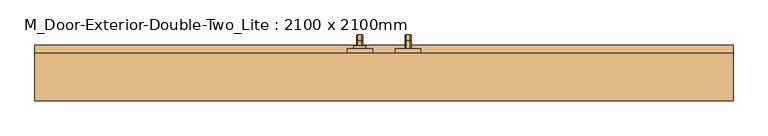
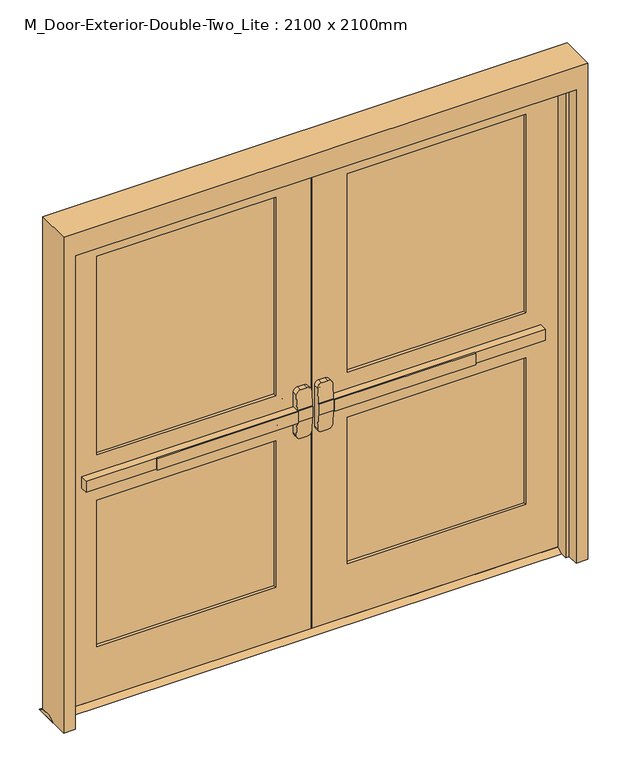
"""IFC4 building model written with IfcOpenShell, lengths in millimetres: door geometry, M_Door-Exterior-Double-Two_Lite : 2100 x 2100mm."""

from ifc_helpers import new_model, si_unit, point, frame, frame_2d, origin, place, context, project, spatial, polyline, circle_curve, ellipse_curve, trimmed, segment, composite_curve, outline, extrude, faceted_brep, source, transform, mapped, element, save
from ifc_brep_helpers import plane_surface, cylinder_surface, revolved_surface, advanced_brep


def m_door_exterior_double_two_lite_2100_x_2100mm_462d4e28(model_context):
    return source(origin(), model_context, "Body", "SolidModel", [
        extrude(outline(polyline([(-667.2, -39.25), (-667.2, -32.9), (-76.2, -32.9), (-76.2, -39.25), (-667.2, -39.25)])), frame((0.0, 0.0, 974.6), z_axis=(0.0, 0.0, 1.0), x_axis=(1.0, 0.0, 0.0)), (0.0, 0.0, 1.0), 50.8),
        advanced_brep(
        [(-12.7, -32.9, 1025.4), (-76.2, -32.9, 1025.4), (-962.7, -32.9, 1025.4), (-962.7, -32.9, 974.6), (-76.2, -32.9, 974.6), (-12.7, -32.9, 974.6), (-962.7, -1.15, 1025.4), (-76.2, -1.15, 1025.4), (-76.2, -1.15, 1088.9), (-57.15, -1.15, 1107.95), (-31.75, -1.15, 1107.95), (-12.7, -1.15, 1088.9), (-12.7, -1.15, 911.1), (-31.75, -1.15, 892.05), (-57.15, -1.15, 892.05), (-76.2, -1.15, 911.1), (-76.2, -1.15, 974.6), (-962.7, -1.15, 974.6), (-12.7, -29.7247533, 1025.4), (-76.2, -29.7247533, 1025.4), (-12.7, -29.7247533, 974.6), (-12.7, -24.7145731, 911.1), (-12.7, -24.7145731, 1088.9), (-76.2, -29.7247533, 974.6), (-76.2, -24.7145731, 1088.9), (-76.2, -24.7145731, 911.1), (-57.15, -23.211519, 1107.95), (-31.75, -23.211519, 1107.95), (-31.75, -23.211519, 892.05), (-57.15, -23.211519, 892.05)],
        [
            (0, 1),
            (1, 2),
            (2, 3),
            (3, 4),
            (4, 5),
            (5, 0),
            (6, 7),
            (7, 8),
            (8, 9, circle_curve(frame((-57.15, -1.15, 1088.9), z_axis=(0.0, 1.0, 0.0), x_axis=(-1.0, 0.0, 0.0)), 19.05)),
            (9, 10),
            (10, 11, circle_curve(frame((-31.75, -1.15, 1088.9), z_axis=(0.0, 1.0, 0.0), x_axis=(-1.0, 0.0, 0.0)), 19.05)),
            (11, 12),
            (12, 13, circle_curve(frame((-31.75, -1.15, 911.1), z_axis=(0.0, 1.0, 0.0), x_axis=(-1.0, 0.0, 0.0)), 19.05)),
            (13, 14),
            (14, 15, circle_curve(frame((-57.15, -1.15, 911.1), z_axis=(0.0, 1.0, 0.0), x_axis=(-1.0, 0.0, 0.0)), 19.05)),
            (15, 16),
            (16, 17),
            (17, 6),
            (0, 18),
            (18, 19),
            (19, 7),
            (6, 2),
            (5, 20),
            (20, 21),
            (21, 12),
            (11, 22),
            (22, 18),
            (16, 23),
            (23, 20),
            (3, 17),
            (19, 24),
            (24, 8),
            (15, 25),
            (25, 23),
            (9, 26),
            (26, 27),
            (27, 10),
            (13, 28),
            (28, 29),
            (29, 14),
            (29, 25, ellipse_curve(frame((-57.15, -24.7145731, 911.1), z_axis=(0.0, 0.9969018152893365, 0.07865602756830282), x_axis=(0.0, -0.07865602756830208, 0.9969018152893365)), 19.1092038, 19.05)),
            (24, 26, ellipse_curve(frame((-57.15, -24.7145731, 1088.9), z_axis=(0.0, 0.9969018152893376, -0.07865602756828934), x_axis=(0.0, -0.078656027568288, -0.9969018152893377)), 19.1092038, 19.05)),
            (27, 22, ellipse_curve(frame((-31.75, -24.7145731, 1088.9), z_axis=(0.0, 0.9969018152893376, -0.07865602756828934), x_axis=(0.0, -0.078656027568288, -0.9969018152893377)), 19.1092038, 19.05)),
            (21, 28, ellipse_curve(frame((-31.75, -24.7145731, 911.1), z_axis=(0.0, 0.9969018152893365, 0.07865602756830282), x_axis=(0.0, -0.07865602756830208, 0.9969018152893365)), 19.1092038, 19.05)),
        ],
        [
            plane_surface(frame((-12.7, -32.9, 1025.4), z_axis=(0.0, -1.0, 0.0), x_axis=(1.0, 0.0, 0.0))),
            plane_surface(frame((-12.7, -1.15, 1025.4), z_axis=(0.0, 1.0, 0.0), x_axis=(-1.0, 0.0, 0.0))),
            plane_surface(frame((-962.7, -32.9, 1025.4), z_axis=(0.0, 0.0, 1.0), x_axis=(0.0, 1.0, 0.0))),
            plane_surface(frame((-12.7, -32.9, 1025.4), z_axis=(1.0, 0.0, 0.0), x_axis=(0.0, 1.0, 0.0))),
            plane_surface(frame((-12.7, -32.9, 974.6), z_axis=(0.0, 0.0, -1.0), x_axis=(0.0, 1.0, 0.0))),
            plane_surface(frame((-962.7, -32.9, 974.6), z_axis=(-1.0, 0.0, 0.0), x_axis=(0.0, 1.0, 0.0))),
            plane_surface(frame((-76.2, -29.7247533, 911.1), z_axis=(-1.0, 0.0, 0.0), x_axis=(0.0, 1.0, 0.0))),
            plane_surface(frame((-57.15, -29.7247533, 1107.95), z_axis=(0.0, 0.0, 1.0), x_axis=(0.0, 1.0, 0.0))),
            plane_surface(frame((-31.75, -29.7247533, 892.05), z_axis=(0.0, 0.0, -1.0), x_axis=(0.0, 1.0, 0.0))),
            cylinder_surface(frame((-57.15, -1.15, 911.1), z_axis=(0.0, -1.0, 0.0), x_axis=(-1.0, 0.0, 0.0)), 19.05),
            cylinder_surface(frame((-57.15, -1.15, 1088.9), z_axis=(0.0, -1.0, 0.0), x_axis=(-1.0, 0.0, 0.0)), 19.05),
            cylinder_surface(frame((-31.75, -1.15, 1088.9), z_axis=(0.0, -1.0, 0.0), x_axis=(-1.0, 0.0, 0.0)), 19.05),
            cylinder_surface(frame((-31.75, -1.15, 911.1), z_axis=(0.0, -1.0, 0.0), x_axis=(-1.0, 0.0, 0.0)), 19.05),
            plane_surface(frame((-76.2, -29.7247533, 1025.4), z_axis=(0.0, -0.9969018152893376, 0.07865602756828934), x_axis=(1.0, 0.0, 0.0))),
            plane_surface(frame((-76.2, -23.211519, 892.05), z_axis=(0.0, -0.9969018152893365, -0.07865602756830282), x_axis=(1.0, 0.0, 0.0))),
        ],
        [
            (0, [[1, 2, 3, 4, 5, 6]]),
            (1, [[7, 8, 9, 10, 11, 12, 13, 14, 15, 16, 17, 18]]),
            (2, [[-2, -1, 19, 20, 21, -7, 22]]),
            (3, [[23, 24, 25, -12, 26, 27, -19, -6]]),
            (4, [[-17, 28, 29, -23, -5, -4, 30]]),
            (5, [[-22, -18, -30, -3]]),
            (6, [[-21, 31, 32, -8]]),
            (6, [[33, 34, -28, -16]]),
            (7, [[35, 36, 37, -10]]),
            (8, [[38, 39, 40, -14]]),
            (9, [[-40, 41, -33, -15]]),
            (10, [[-32, 42, -35, -9]]),
            (11, [[-37, 43, -26, -11]]),
            (12, [[-25, 44, -38, -13]]),
            (13, [[-27, -43, -36, -42, -31, -20]]),
            (14, [[-29, -34, -41, -39, -44, -24]]),
        ],
    ),
        extrude(outline(polyline([(43.85, 15.0), (69.25, 0.0), (-26.55, 0.0), (-1.15, 15.0), (43.85, 15.0)])), frame((-1100.0, 0.0, 0.0), z_axis=(1.0, 0.0, 0.0), x_axis=(0.0, 1.0, 0.0)), (0.0, 0.0, 1.0), 2200.0),
        extrude(outline(polyline([(667.2, -39.25), (76.2, -39.25), (76.2, -32.9), (667.2, -32.9), (667.2, -39.25)])), frame((0.0, 0.0, 974.6), z_axis=(0.0, 0.0, 1.0), x_axis=(1.0, 0.0, 0.0)), (0.0, 0.0, 1.0), 50.8),
        advanced_brep(
        [(12.7, -32.9, 1025.4), (12.7, -32.9, 974.6), (76.2, -32.9, 974.6), (962.7, -32.9, 974.6), (962.7, -32.9, 1025.4), (76.2, -32.9, 1025.4), (962.7, -1.15, 1025.4), (962.7, -1.15, 974.6), (76.2, -1.15, 974.6), (76.2, -1.15, 911.1), (57.15, -1.15, 892.05), (31.75, -1.15, 892.05), (12.7, -1.15, 911.1), (12.7, -1.15, 1088.9), (31.75, -1.15, 1107.95), (57.15, -1.15, 1107.95), (76.2, -1.15, 1088.9), (76.2, -1.15, 1025.4), (76.2, -29.7247533, 1025.4), (12.7, -29.7247533, 1025.4), (12.7, -24.7145731, 1088.9), (12.7, -24.7145731, 911.1), (12.7, -29.7247533, 974.6), (76.2, -29.7247533, 974.6), (76.2, -24.7145731, 911.1), (76.2, -24.7145731, 1088.9), (31.75, -23.211519, 1107.95), (57.15, -23.211519, 1107.95), (57.15, -23.211519, 892.05), (31.75, -23.211519, 892.05)],
        [
            (0, 1),
            (1, 2),
            (2, 3),
            (3, 4),
            (4, 5),
            (5, 0),
            (6, 7),
            (7, 8),
            (8, 9),
            (9, 10, circle_curve(frame((57.15, -1.15, 911.1), z_axis=(0.0, 1.0, 0.0), x_axis=(1.0, 0.0, 0.0)), 19.05)),
            (10, 11),
            (11, 12, circle_curve(frame((31.75, -1.15, 911.1), z_axis=(0.0, 1.0, 0.0), x_axis=(1.0, 0.0, 0.0)), 19.05)),
            (12, 13),
            (13, 14, circle_curve(frame((31.75, -1.15, 1088.9), z_axis=(0.0, 1.0, 0.0), x_axis=(1.0, 0.0, 0.0)), 19.05)),
            (14, 15),
            (15, 16, circle_curve(frame((57.15, -1.15, 1088.9), z_axis=(0.0, 1.0, 0.0), x_axis=(1.0, 0.0, 0.0)), 19.05)),
            (16, 17),
            (17, 6),
            (4, 6),
            (17, 18),
            (18, 19),
            (19, 0),
            (19, 20),
            (20, 13),
            (12, 21),
            (21, 22),
            (22, 1),
            (7, 3),
            (22, 23),
            (23, 8),
            (23, 24),
            (24, 9),
            (16, 25),
            (25, 18),
            (14, 26),
            (26, 27),
            (27, 15),
            (10, 28),
            (28, 29),
            (29, 11),
            (24, 28, ellipse_curve(frame((57.15, -24.7145731, 911.1), z_axis=(0.0, 0.9969018152893365, 0.07865602756830282), x_axis=(0.0, -0.07865602756830208, 0.9969018152893365)), 19.1092038, 19.05)),
            (27, 25, ellipse_curve(frame((57.15, -24.7145731, 1088.9), z_axis=(0.0, 0.9969018152893376, -0.07865602756828934), x_axis=(0.0, -0.078656027568288, -0.9969018152893377)), 19.1092038, 19.05)),
            (20, 26, ellipse_curve(frame((31.75, -24.7145731, 1088.9), z_axis=(0.0, 0.9969018152893376, -0.07865602756828934), x_axis=(0.0, -0.078656027568288, -0.9969018152893377)), 19.1092038, 19.05)),
            (29, 21, ellipse_curve(frame((31.75, -24.7145731, 911.1), z_axis=(0.0, 0.9969018152893365, 0.07865602756830282), x_axis=(0.0, -0.07865602756830208, 0.9969018152893365)), 19.1092038, 19.05)),
        ],
        [
            plane_surface(frame((12.7, -32.9, 1025.4), z_axis=(0.0, -1.0, 0.0), x_axis=(-1.0, 0.0, 0.0))),
            plane_surface(frame((12.7, -1.15, 1025.4), z_axis=(0.0, 1.0, 0.0), x_axis=(1.0, 0.0, 0.0))),
            plane_surface(frame((962.7, -32.9, 1025.4), z_axis=(0.0, 0.0, 1.0), x_axis=(0.0, 1.0, 0.0))),
            plane_surface(frame((12.7, -32.9, 1025.4), z_axis=(-1.0, 0.0, 0.0), x_axis=(0.0, 1.0, 0.0))),
            plane_surface(frame((12.7, -32.9, 974.6), z_axis=(0.0, 0.0, -1.0), x_axis=(0.0, 1.0, 0.0))),
            plane_surface(frame((962.7, -32.9, 974.6), z_axis=(1.0, 0.0, 0.0), x_axis=(0.0, 1.0, 0.0))),
            plane_surface(frame((76.2, -29.7247533, 911.1), z_axis=(1.0, 0.0, 0.0), x_axis=(0.0, 1.0, 0.0))),
            plane_surface(frame((57.15, -29.7247533, 1107.95), z_axis=(0.0, 0.0, 1.0), x_axis=(0.0, 1.0, 0.0))),
            plane_surface(frame((31.75, -29.7247533, 892.05), z_axis=(0.0, 0.0, -1.0), x_axis=(0.0, 1.0, 0.0))),
            cylinder_surface(frame((57.15, -1.15, 911.1), z_axis=(0.0, -1.0, 0.0), x_axis=(1.0, 0.0, 0.0)), 19.05),
            cylinder_surface(frame((57.15, -1.15, 1088.9), z_axis=(0.0, -1.0, 0.0), x_axis=(1.0, 0.0, 0.0)), 19.05),
            cylinder_surface(frame((31.75, -1.15, 1088.9), z_axis=(0.0, -1.0, 0.0), x_axis=(1.0, 0.0, 0.0)), 19.05),
            cylinder_surface(frame((31.75, -1.15, 911.1), z_axis=(0.0, -1.0, 0.0), x_axis=(1.0, 0.0, 0.0)), 19.05),
            plane_surface(frame((76.2, -29.7247533, 1025.4), z_axis=(0.0, -0.9969018152893376, 0.07865602756828934), x_axis=(-1.0, 0.0, 0.0))),
            plane_surface(frame((76.2, -23.211519, 892.05), z_axis=(0.0, -0.9969018152893365, -0.07865602756830282), x_axis=(-1.0, 0.0, 0.0))),
        ],
        [
            (0, [[1, 2, 3, 4, 5, 6]]),
            (1, [[7, 8, 9, 10, 11, 12, 13, 14, 15, 16, 17, 18]]),
            (2, [[19, -18, 20, 21, 22, -6, -5]]),
            (3, [[-1, -22, 23, 24, -13, 25, 26, 27]]),
            (4, [[28, -3, -2, -27, 29, 30, -8]]),
            (5, [[-4, -28, -7, -19]]),
            (6, [[-9, -30, 31, 32]]),
            (6, [[-17, 33, 34, -20]]),
            (7, [[-15, 35, 36, 37]]),
            (8, [[-11, 38, 39, 40]]),
            (9, [[-10, -32, 41, -38]]),
            (10, [[-16, -37, 42, -33]]),
            (11, [[-14, -24, 43, -35]]),
            (12, [[-12, -40, 44, -25]]),
            (13, [[-21, -34, -42, -36, -43, -23]]),
            (14, [[-26, -44, -39, -41, -31, -29]]),
        ],
    ),
        advanced_brep(
        [(66.2, 58.85, 1001.190625), (66.2, 58.85, 998.809375), (69.771875, 58.85, 995.2375), (82.6284594, 58.85, 995.2375), (86.2, 58.85, 998.8090406), (86.2, 58.85, 1001.190625), (82.628125, 58.85, 1004.7625), (69.771875, 58.85, 1004.7625), (66.2, 58.85, 874.609375), (69.771875, 58.85, 871.0375), (82.628125, 58.85, 871.0375), (86.2, 58.85, 874.609375), (86.2, 58.85, 876.9909594), (82.6284594, 58.85, 880.5625), (69.771875, 58.85, 880.5625), (66.2, 58.85, 876.990625), (66.2, 84.25, 1001.190625), (66.2, 98.140625, 987.3), (66.2, 98.140625, 888.5), (66.2, 84.25, 874.609375), (66.2, 84.25, 876.990625), (66.2, 95.759375, 888.5), (66.2, 95.759375, 987.3), (66.2, 84.25, 998.809375), (69.771875, 84.25, 995.2375), (82.6284594, 84.25, 995.2375), (86.2, 84.25, 998.8090406), (86.2, 95.7590406, 987.3), (86.2, 95.7590406, 888.5), (86.2, 84.25, 876.9909594), (86.2, 84.25, 874.609375), (86.2, 98.140625, 888.5), (86.2, 98.140625, 987.3), (86.2, 84.25, 1001.190625), (82.628125, 84.25, 1004.7625), (69.771875, 84.25, 1004.7625), (69.771875, 92.1875, 987.3), (82.6284594, 92.1875, 987.3), (82.628125, 101.7125, 987.3), (69.771875, 101.7125, 987.3), (69.771875, 92.1875, 888.5), (82.6284594, 92.1875, 888.5), (82.628125, 101.7125, 888.5), (69.771875, 101.7125, 888.5), (69.771875, 84.25, 880.5625), (82.6284594, 84.25, 880.5625), (82.628125, 84.25, 871.0375), (69.771875, 84.25, 871.0375)],
        [
            (0, 1),
            (1, 2, circle_curve(frame((69.771875, 58.85, 998.809375), z_axis=(0.0, -1.0, 0.0), x_axis=(0.0, 0.0, 1.0)), 3.571875)),
            (2, 3),
            (3, 4, circle_curve(frame((82.6284594, 58.85, 998.8090406), z_axis=(0.0, -1.0, 0.0), x_axis=(0.0, 0.0, 1.0)), 3.5715406)),
            (4, 5),
            (5, 6, circle_curve(frame((82.628125, 58.85, 1001.190625), z_axis=(0.0, -1.0, 0.0), x_axis=(0.0, 0.0, 1.0)), 3.571875)),
            (6, 7),
            (7, 0, circle_curve(frame((69.771875, 58.85, 1001.190625), z_axis=(0.0, -1.0, 0.0), x_axis=(0.0, 0.0, 1.0)), 3.571875)),
            (8, 9, circle_curve(frame((69.771875, 58.85, 874.609375), z_axis=(0.0, -1.0, 0.0), x_axis=(0.0, 0.0, -1.0)), 3.571875)),
            (9, 10),
            (10, 11, circle_curve(frame((82.628125, 58.85, 874.609375), z_axis=(0.0, -1.0, 0.0), x_axis=(0.0, 0.0, -1.0)), 3.571875)),
            (11, 12),
            (12, 13, circle_curve(frame((82.6284594, 58.85, 876.9909594), z_axis=(0.0, -1.0, 0.0), x_axis=(0.0, 0.0, -1.0)), 3.5715406)),
            (13, 14),
            (14, 15, circle_curve(frame((69.771875, 58.85, 876.990625), z_axis=(0.0, -1.0, 0.0), x_axis=(0.0, 0.0, -1.0)), 3.571875)),
            (15, 8),
            (0, 16),
            (16, 17, circle_curve(frame((66.2, 84.25, 987.3), z_axis=(-1.0, 0.0, 0.0), x_axis=(0.0, 0.0, 1.0)), 13.890625)),
            (17, 18),
            (18, 19, circle_curve(frame((66.2, 84.25, 888.5), z_axis=(-1.0, 0.0, 0.0), x_axis=(0.0, 1.0, 0.0)), 13.890625)),
            (19, 8),
            (15, 20),
            (20, 21, circle_curve(frame((66.2, 84.25, 888.5), z_axis=(1.0, 0.0, 0.0), x_axis=(0.0, 1.0, 0.0)), 11.509375)),
            (21, 22),
            (22, 23, circle_curve(frame((66.2, 84.25, 987.3), z_axis=(1.0, 0.0, 0.0), x_axis=(0.0, 0.0, 1.0)), 11.509375)),
            (23, 1),
            (23, 24, circle_curve(frame((69.771875, 84.25, 998.809375), z_axis=(0.0, -1.0, 0.0), x_axis=(0.0, 0.0, 1.0)), 3.571875)),
            (24, 2),
            (24, 25),
            (25, 3),
            (25, 26, circle_curve(frame((82.6284594, 84.25, 998.8090406), z_axis=(0.0, -1.0, 0.0), x_axis=(0.0, 0.0, 1.0)), 3.5715406)),
            (26, 4),
            (26, 27, circle_curve(frame((86.2, 84.25, 987.3), z_axis=(-1.0, 0.0, 0.0), x_axis=(0.0, 0.0, 1.0)), 11.5090406)),
            (27, 28),
            (28, 29, circle_curve(frame((86.2, 84.25, 888.5), z_axis=(-1.0, 0.0, 0.0), x_axis=(0.0, 1.0, 0.0)), 11.5090406)),
            (29, 12),
            (11, 30),
            (30, 31, circle_curve(frame((86.2, 84.25, 888.5), z_axis=(1.0, 0.0, 0.0), x_axis=(0.0, 1.0, 0.0)), 13.890625)),
            (31, 32),
            (32, 33, circle_curve(frame((86.2, 84.25, 987.3), z_axis=(1.0, 0.0, 0.0), x_axis=(0.0, 0.0, 1.0)), 13.890625)),
            (33, 5),
            (33, 34, circle_curve(frame((82.628125, 84.25, 1001.190625), z_axis=(0.0, -1.0, 0.0), x_axis=(0.0, 0.0, 1.0)), 3.571875)),
            (34, 6),
            (34, 35),
            (35, 7),
            (35, 16, circle_curve(frame((69.771875, 84.25, 1001.190625), z_axis=(0.0, -1.0, 0.0), x_axis=(0.0, 0.0, 1.0)), 3.571875)),
            (36, 24, circle_curve(frame((69.771875, 84.25, 987.3), z_axis=(1.0, 0.0, 0.0), x_axis=(0.0, 0.0, 1.0)), 7.9375)),
            (22, 36, circle_curve(frame((69.771875, 95.759375, 987.3), z_axis=(0.0, 0.0, 1.0), x_axis=(0.0, 1.0, 0.0)), 3.571875)),
            (37, 25, circle_curve(frame((82.6284594, 84.25, 987.3), z_axis=(1.0, 0.0, 0.0), x_axis=(0.0, 0.0, 1.0)), 7.9375)),
            (36, 37),
            (37, 27, circle_curve(frame((82.6284594, 95.7590406, 987.3), z_axis=(0.0, 0.0, 1.0), x_axis=(0.0, 1.0, 0.0)), 3.5715406)),
            (38, 34, circle_curve(frame((82.628125, 84.25, 987.3), z_axis=(1.0, 0.0, 0.0), x_axis=(0.0, 0.0, 1.0)), 17.4625)),
            (32, 38, circle_curve(frame((82.628125, 98.140625, 987.3), z_axis=(0.0, 0.0, 1.0), x_axis=(0.0, 1.0, 0.0)), 3.571875)),
            (39, 35, circle_curve(frame((69.771875, 84.25, 987.3), z_axis=(1.0, 0.0, 0.0), x_axis=(0.0, 0.0, 1.0)), 17.4625)),
            (38, 39),
            (39, 17, circle_curve(frame((69.771875, 98.140625, 987.3), z_axis=(0.0, 0.0, 1.0), x_axis=(0.0, 1.0, 0.0)), 3.571875)),
            (21, 40, circle_curve(frame((69.771875, 95.759375, 888.5), z_axis=(0.0, 0.0, 1.0), x_axis=(0.0, 1.0, 0.0)), 3.571875)),
            (40, 36),
            (40, 41),
            (41, 37),
            (41, 28, circle_curve(frame((82.6284594, 95.7590406, 888.5), z_axis=(0.0, 0.0, 1.0), x_axis=(0.0, 1.0, 0.0)), 3.5715406)),
            (31, 42, circle_curve(frame((82.628125, 98.140625, 888.5), z_axis=(0.0, 0.0, 1.0), x_axis=(0.0, 1.0, 0.0)), 3.571875)),
            (42, 38),
            (42, 43),
            (43, 39),
            (43, 18, circle_curve(frame((69.771875, 98.140625, 888.5), z_axis=(0.0, 0.0, 1.0), x_axis=(0.0, 1.0, 0.0)), 3.571875)),
            (44, 40, circle_curve(frame((69.771875, 84.25, 888.5), z_axis=(1.0, 0.0, 0.0), x_axis=(0.0, 1.0, 0.0)), 7.9375)),
            (20, 44, circle_curve(frame((69.771875, 84.25, 876.990625), z_axis=(0.0, 1.0, 0.0), x_axis=(0.0, 0.0, -1.0)), 3.571875)),
            (45, 41, circle_curve(frame((82.6284594, 84.25, 888.5), z_axis=(1.0, 0.0, 0.0), x_axis=(0.0, 1.0, 0.0)), 7.9375)),
            (44, 45),
            (45, 29, circle_curve(frame((82.6284594, 84.25, 876.9909594), z_axis=(0.0, 1.0, 0.0), x_axis=(0.0, 0.0, -1.0)), 3.5715406)),
            (46, 42, circle_curve(frame((82.628125, 84.25, 888.5), z_axis=(1.0, 0.0, 0.0), x_axis=(0.0, 1.0, 0.0)), 17.4625)),
            (30, 46, circle_curve(frame((82.628125, 84.25, 874.609375), z_axis=(0.0, 1.0, 0.0), x_axis=(0.0, 0.0, -1.0)), 3.571875)),
            (47, 43, circle_curve(frame((69.771875, 84.25, 888.5), z_axis=(1.0, 0.0, 0.0), x_axis=(0.0, 1.0, 0.0)), 17.4625)),
            (46, 47),
            (47, 19, circle_curve(frame((69.771875, 84.25, 874.609375), z_axis=(0.0, 1.0, 0.0), x_axis=(0.0, 0.0, -1.0)), 3.571875)),
            (14, 44),
            (13, 45),
            (10, 46),
            (9, 47),
        ],
        [
            plane_surface(frame((76.2, 58.85, 1000.0), z_axis=(0.0, -1.0, 0.0), x_axis=(1.0, 0.0, 0.0))),
            plane_surface(frame((76.2, 58.85, 875.8), z_axis=(0.0, -1.0, 0.0), x_axis=(1.0, 0.0, 0.0))),
            plane_surface(frame((66.2, 58.85, 1001.190625), z_axis=(-1.0, 0.0, 0.0), x_axis=(0.0, 1.0, 0.0))),
            cylinder_surface(frame((69.771875, 58.85, 998.809375), z_axis=(0.0, -1.0, 0.0), x_axis=(0.0, 0.0, 1.0)), 3.571875),
            plane_surface(frame((69.771875, 58.85, 995.2375), z_axis=(0.0, 0.0, -1.0), x_axis=(0.0, 1.0, 0.0))),
            cylinder_surface(frame((82.6284594, 58.85, 998.8090406), z_axis=(0.0, -1.0, 0.0), x_axis=(0.0, 0.0, 1.0)), 3.5715406),
            plane_surface(frame((86.2, 58.85, 998.8090406), z_axis=(1.0, 0.0, 0.0), x_axis=(0.0, 1.0, 0.0))),
            cylinder_surface(frame((82.628125, 58.85, 1001.190625), z_axis=(0.0, -1.0, 0.0), x_axis=(0.0, 0.0, 1.0)), 3.571875),
            plane_surface(frame((82.628125, 58.85, 1004.7625), z_axis=(0.0, 0.0, 1.0), x_axis=(0.0, 1.0, 0.0))),
            cylinder_surface(frame((69.771875, 58.85, 1001.190625), z_axis=(0.0, -1.0, 0.0), x_axis=(0.0, 0.0, 1.0)), 3.571875),
            revolved_surface(trimmed(ellipse_curve(frame((69.771875, 84.25, 998.809375), z_axis=(0.0, -1.0, 0.0), x_axis=(0.0, 0.0, 1.0)), 3.571875, 3.571875), [point((66.2, 84.25, 998.809375))], [point((69.771875, 84.25, 995.2375))], True, "CARTESIAN"), (76.2, 84.25, 987.3), (-1.0, 0.0, 0.0)),
            revolved_surface(polyline([(69.771875, 84.25, 995.2375), (82.6284594, 84.25, 995.2375)]), (76.2, 84.25, 987.3), (-1.0, 0.0, 0.0)),
            revolved_surface(trimmed(ellipse_curve(frame((82.6284594, 84.25, 998.8090406), z_axis=(0.0, -1.0, 0.0), x_axis=(0.0, 0.0, 1.0)), 3.5715406, 3.5715406), [point((82.6284594, 84.25, 995.2375))], [point((86.2, 84.25, 998.8090406))], True, "CARTESIAN"), (76.2, 84.25, 987.3), (-1.0, 0.0, 0.0)),
            revolved_surface(trimmed(ellipse_curve(frame((82.628125, 84.25, 1001.190625), z_axis=(0.0, -1.0, 0.0), x_axis=(0.0, 0.0, 1.0)), 3.571875, 3.571875), [point((86.2, 84.25, 1001.190625))], [point((82.628125, 84.25, 1004.7625))], True, "CARTESIAN"), (76.2, 84.25, 987.3), (-1.0, 0.0, 0.0)),
            cylinder_surface(frame((76.2, 84.25, 987.3), z_axis=(-1.0, 0.0, 0.0), x_axis=(0.0, 0.0, 1.0)), 17.4625),
            revolved_surface(trimmed(ellipse_curve(frame((69.771875, 84.25, 1001.190625), z_axis=(0.0, -1.0, 0.0), x_axis=(0.0, 0.0, 1.0)), 3.571875, 3.571875), [point((69.771875, 84.25, 1004.7625))], [point((66.2, 84.25, 1001.190625))], True, "CARTESIAN"), (76.2, 84.25, 987.3), (-1.0, 0.0, 0.0)),
            cylinder_surface(frame((69.771875, 95.759375, 987.3), z_axis=(0.0, 0.0, 1.0), x_axis=(0.0, 1.0, 0.0)), 3.571875),
            plane_surface(frame((69.771875, 92.1875, 987.3), z_axis=(0.0, -1.0, 0.0), x_axis=(0.0, 0.0, -1.0))),
            cylinder_surface(frame((82.6284594, 95.7590406, 987.3), z_axis=(0.0, 0.0, 1.0), x_axis=(0.0, 1.0, 0.0)), 3.5715406),
            cylinder_surface(frame((82.628125, 98.140625, 987.3), z_axis=(0.0, 0.0, 1.0), x_axis=(0.0, 1.0, 0.0)), 3.571875),
            plane_surface(frame((82.628125, 101.7125, 987.3), z_axis=(0.0, 1.0, 0.0), x_axis=(0.0, 0.0, -1.0))),
            cylinder_surface(frame((69.771875, 98.140625, 987.3), z_axis=(0.0, 0.0, 1.0), x_axis=(0.0, 1.0, 0.0)), 3.571875),
            revolved_surface(trimmed(ellipse_curve(frame((69.771875, 95.759375, 888.5), z_axis=(0.0, 0.0, 1.0), x_axis=(0.0, 1.0, 0.0)), 3.571875, 3.571875), [point((66.2, 95.759375, 888.5))], [point((69.771875, 92.1875, 888.5))], True, "CARTESIAN"), (76.2, 84.25, 888.5), (-1.0, 0.0, 0.0)),
            revolved_surface(polyline([(69.771875, 92.1875, 888.5), (82.6284594, 92.1875, 888.5)]), (76.2, 84.25, 888.5), (-1.0, 0.0, 0.0)),
            revolved_surface(trimmed(ellipse_curve(frame((82.6284594, 95.7590406, 888.5), z_axis=(0.0, 0.0, 1.0), x_axis=(0.0, 1.0, 0.0)), 3.5715406, 3.5715406), [point((82.6284594, 92.1875, 888.5))], [point((86.2, 95.7590406, 888.5))], True, "CARTESIAN"), (76.2, 84.25, 888.5), (-1.0, 0.0, 0.0)),
            revolved_surface(trimmed(ellipse_curve(frame((82.628125, 98.140625, 888.5), z_axis=(0.0, 0.0, 1.0), x_axis=(0.0, 1.0, 0.0)), 3.571875, 3.571875), [point((86.2, 98.140625, 888.5))], [point((82.628125, 101.7125, 888.5))], True, "CARTESIAN"), (76.2, 84.25, 888.5), (-1.0, 0.0, 0.0)),
            cylinder_surface(frame((76.2, 84.25, 888.5), z_axis=(-1.0, 0.0, 0.0), x_axis=(0.0, 1.0, 0.0)), 17.4625),
            revolved_surface(trimmed(ellipse_curve(frame((69.771875, 98.140625, 888.5), z_axis=(0.0, 0.0, 1.0), x_axis=(0.0, 1.0, 0.0)), 3.571875, 3.571875), [point((69.771875, 101.7125, 888.5))], [point((66.2, 98.140625, 888.5))], True, "CARTESIAN"), (76.2, 84.25, 888.5), (-1.0, 0.0, 0.0)),
            cylinder_surface(frame((69.771875, 84.25, 876.990625), z_axis=(0.0, 1.0, 0.0), x_axis=(0.0, 0.0, -1.0)), 3.571875),
            plane_surface(frame((69.771875, 84.25, 880.5625), z_axis=(0.0, 0.0, 1.0), x_axis=(0.0, -1.0, 0.0))),
            cylinder_surface(frame((82.6284594, 84.25, 876.9909594), z_axis=(0.0, 1.0, 0.0), x_axis=(0.0, 0.0, -1.0)), 3.5715406),
            cylinder_surface(frame((82.628125, 84.25, 874.609375), z_axis=(0.0, 1.0, 0.0), x_axis=(0.0, 0.0, -1.0)), 3.571875),
            plane_surface(frame((82.628125, 84.25, 871.0375), z_axis=(0.0, 0.0, -1.0), x_axis=(0.0, -1.0, 0.0))),
            cylinder_surface(frame((69.771875, 84.25, 874.609375), z_axis=(0.0, 1.0, 0.0), x_axis=(0.0, 0.0, -1.0)), 3.571875),
        ],
        [
            (0, [[1, 2, 3, 4, 5, 6, 7, 8]]),
            (1, [[9, 10, 11, 12, 13, 14, 15, 16]]),
            (2, [[-1, 17, 18, 19, 20, 21, -16, 22, 23, 24, 25, 26]]),
            (3, [[-2, -26, 27, 28]]),
            (4, [[-3, -28, 29, 30]]),
            (5, [[-4, -30, 31, 32]]),
            (6, [[-5, -32, 33, 34, 35, 36, -12, 37, 38, 39, 40, 41]]),
            (7, [[-6, -41, 42, 43]]),
            (8, [[-7, -43, 44, 45]]),
            (9, [[-8, -45, 46, -17]]),
            (10, [[47, -27, -25, 48]]),
            (11, [[49, -29, -47, 50]]),
            (12, [[-33, -31, -49, 51]]),
            (13, [[52, -42, -40, 53]]),
            (14, [[54, -44, -52, 55]]),
            (15, [[-18, -46, -54, 56]]),
            (16, [[-48, -24, 57, 58]]),
            (17, [[-50, -58, 59, 60]]),
            (18, [[-51, -60, 61, -34]]),
            (19, [[-53, -39, 62, 63]]),
            (20, [[-55, -63, 64, 65]]),
            (21, [[-56, -65, 66, -19]]),
            (22, [[67, -57, -23, 68]]),
            (23, [[69, -59, -67, 70]]),
            (24, [[-35, -61, -69, 71]]),
            (25, [[72, -62, -38, 73]]),
            (26, [[74, -64, -72, 75]]),
            (27, [[-20, -66, -74, 76]]),
            (28, [[-68, -22, -15, 77]]),
            (29, [[-70, -77, -14, 78]]),
            (30, [[-71, -78, -13, -36]]),
            (31, [[-73, -37, -11, 79]]),
            (32, [[-75, -79, -10, 80]]),
            (33, [[-76, -80, -9, -21]]),
        ],
    ),
        extrude(outline(composite_curve([segment(trimmed(circle_curve(frame_2d((1094.2338574, 76.2)), 90.1286291), [point((1175.0, 116.2))], [point((1175.0, 36.2))], False, "CARTESIAN"), True, "CONTINUOUS"), segment(polyline([(1175.0, 36.2), (825.0, 36.2)]), True, "CONTINUOUS"), segment(trimmed(circle_curve(frame_2d((905.7661426, 76.2)), 90.1286291), [point((825.0, 36.2))], [point((825.0, 116.2))], False, "CARTESIAN"), True, "CONTINUOUS"), segment(polyline([(825.0, 116.2), (1175.0, 116.2)]), True, "CONTINUOUS")], self_intersect=False)), frame((0.0, 43.85, 0.0), z_axis=(0.0, 1.0, 0.0), x_axis=(0.0, 0.0, 1.0)), (0.0, 0.0, 1.0), 15.0),
        advanced_brep(
        [(-86.2, 58.85, 1001.190625), (-86.2, 58.85, 998.809375), (-82.628125, 58.85, 995.2375), (-69.7715406, 58.85, 995.2375), (-66.2, 58.85, 998.8090406), (-66.2, 58.85, 1001.190625), (-69.771875, 58.85, 1004.7625), (-82.628125, 58.85, 1004.7625), (-86.2, 58.85, 874.609375), (-82.628125, 58.85, 871.0375), (-69.771875, 58.85, 871.0375), (-66.2, 58.85, 874.609375), (-66.2, 58.85, 876.9909594), (-69.7715406, 58.85, 880.5625), (-82.628125, 58.85, 880.5625), (-86.2, 58.85, 876.990625), (-86.2, 84.25, 1001.190625), (-86.2, 98.140625, 987.3), (-86.2, 98.140625, 888.5), (-86.2, 84.25, 874.609375), (-86.2, 84.25, 876.990625), (-86.2, 95.759375, 888.5), (-86.2, 95.759375, 987.3), (-86.2, 84.25, 998.809375), (-82.628125, 84.25, 995.2375), (-69.7715406, 84.25, 995.2375), (-66.2, 84.25, 998.8090406), (-66.2, 95.7590406, 987.3), (-66.2, 95.7590406, 888.5), (-66.2, 84.25, 876.9909594), (-66.2, 84.25, 874.609375), (-66.2, 98.140625, 888.5), (-66.2, 98.140625, 987.3), (-66.2, 84.25, 1001.190625), (-69.771875, 84.25, 1004.7625), (-82.628125, 84.25, 1004.7625), (-82.628125, 92.1875, 987.3), (-69.7715406, 92.1875, 987.3), (-69.771875, 101.7125, 987.3), (-82.628125, 101.7125, 987.3), (-82.628125, 92.1875, 888.5), (-69.7715406, 92.1875, 888.5), (-69.771875, 101.7125, 888.5), (-82.628125, 101.7125, 888.5), (-82.628125, 84.25, 880.5625), (-69.7715406, 84.25, 880.5625), (-69.771875, 84.25, 871.0375), (-82.628125, 84.25, 871.0375)],
        [
            (0, 1),
            (1, 2, circle_curve(frame((-82.628125, 58.85, 998.809375), z_axis=(0.0, -1.0, 0.0), x_axis=(0.0, 0.0, 1.0)), 3.571875)),
            (2, 3),
            (3, 4, circle_curve(frame((-69.7715406, 58.85, 998.8090406), z_axis=(0.0, -1.0, 0.0), x_axis=(0.0, 0.0, 1.0)), 3.5715406)),
            (4, 5),
            (5, 6, circle_curve(frame((-69.771875, 58.85, 1001.190625), z_axis=(0.0, -1.0, 0.0), x_axis=(0.0, 0.0, 1.0)), 3.571875)),
            (6, 7),
            (7, 0, circle_curve(frame((-82.628125, 58.85, 1001.190625), z_axis=(0.0, -1.0, 0.0), x_axis=(0.0, 0.0, 1.0)), 3.571875)),
            (8, 9, circle_curve(frame((-82.628125, 58.85, 874.609375), z_axis=(0.0, -1.0, 0.0), x_axis=(0.0, 0.0, -1.0)), 3.571875)),
            (9, 10),
            (10, 11, circle_curve(frame((-69.771875, 58.85, 874.609375), z_axis=(0.0, -1.0, 0.0), x_axis=(0.0, 0.0, -1.0)), 3.571875)),
            (11, 12),
            (12, 13, circle_curve(frame((-69.7715406, 58.85, 876.9909594), z_axis=(0.0, -1.0, 0.0), x_axis=(0.0, 0.0, -1.0)), 3.5715406)),
            (13, 14),
            (14, 15, circle_curve(frame((-82.628125, 58.85, 876.990625), z_axis=(0.0, -1.0, 0.0), x_axis=(0.0, 0.0, -1.0)), 3.571875)),
            (15, 8),
            (0, 16),
            (16, 17, circle_curve(frame((-86.2, 84.25, 987.3), z_axis=(-1.0, 0.0, 0.0), x_axis=(0.0, 0.0, 1.0)), 13.890625)),
            (17, 18),
            (18, 19, circle_curve(frame((-86.2, 84.25, 888.5), z_axis=(-1.0, 0.0, 0.0), x_axis=(0.0, 1.0, 0.0)), 13.890625)),
            (19, 8),
            (15, 20),
            (20, 21, circle_curve(frame((-86.2, 84.25, 888.5), z_axis=(1.0, 0.0, 0.0), x_axis=(0.0, 1.0, 0.0)), 11.509375)),
            (21, 22),
            (22, 23, circle_curve(frame((-86.2, 84.25, 987.3), z_axis=(1.0, 0.0, 0.0), x_axis=(0.0, 0.0, 1.0)), 11.509375)),
            (23, 1),
            (23, 24, circle_curve(frame((-82.628125, 84.25, 998.809375), z_axis=(0.0, -1.0, 0.0), x_axis=(0.0, 0.0, 1.0)), 3.571875)),
            (24, 2),
            (24, 25),
            (25, 3),
            (25, 26, circle_curve(frame((-69.7715406, 84.25, 998.8090406), z_axis=(0.0, -1.0, 0.0), x_axis=(0.0, 0.0, 1.0)), 3.5715406)),
            (26, 4),
            (26, 27, circle_curve(frame((-66.2, 84.25, 987.3), z_axis=(-1.0, 0.0, 0.0), x_axis=(0.0, 0.0, 1.0)), 11.5090406)),
            (27, 28),
            (28, 29, circle_curve(frame((-66.2, 84.25, 888.5), z_axis=(-1.0, 0.0, 0.0), x_axis=(0.0, 1.0, 0.0)), 11.5090406)),
            (29, 12),
            (11, 30),
            (30, 31, circle_curve(frame((-66.2, 84.25, 888.5), z_axis=(1.0, 0.0, 0.0), x_axis=(0.0, 1.0, 0.0)), 13.890625)),
            (31, 32),
            (32, 33, circle_curve(frame((-66.2, 84.25, 987.3), z_axis=(1.0, 0.0, 0.0), x_axis=(0.0, 0.0, 1.0)), 13.890625)),
            (33, 5),
            (33, 34, circle_curve(frame((-69.771875, 84.25, 1001.190625), z_axis=(0.0, -1.0, 0.0), x_axis=(0.0, 0.0, 1.0)), 3.571875)),
            (34, 6),
            (34, 35),
            (35, 7),
            (35, 16, circle_curve(frame((-82.628125, 84.25, 1001.190625), z_axis=(0.0, -1.0, 0.0), x_axis=(0.0, 0.0, 1.0)), 3.571875)),
            (36, 24, circle_curve(frame((-82.628125, 84.25, 987.3), z_axis=(1.0, 0.0, 0.0), x_axis=(0.0, 0.0, 1.0)), 7.9375)),
            (22, 36, circle_curve(frame((-82.628125, 95.759375, 987.3), z_axis=(0.0, 0.0, 1.0), x_axis=(0.0, 1.0, 0.0)), 3.571875)),
            (37, 25, circle_curve(frame((-69.7715406, 84.25, 987.3), z_axis=(1.0, 0.0, 0.0), x_axis=(0.0, 0.0, 1.0)), 7.9375)),
            (36, 37),
            (37, 27, circle_curve(frame((-69.7715406, 95.7590406, 987.3), z_axis=(0.0, 0.0, 1.0), x_axis=(0.0, 1.0, 0.0)), 3.5715406)),
            (38, 34, circle_curve(frame((-69.771875, 84.25, 987.3), z_axis=(1.0, 0.0, 0.0), x_axis=(0.0, 0.0, 1.0)), 17.4625)),
            (32, 38, circle_curve(frame((-69.771875, 98.140625, 987.3), z_axis=(0.0, 0.0, 1.0), x_axis=(0.0, 1.0, 0.0)), 3.571875)),
            (39, 35, circle_curve(frame((-82.628125, 84.25, 987.3), z_axis=(1.0, 0.0, 0.0), x_axis=(0.0, 0.0, 1.0)), 17.4625)),
            (38, 39),
            (39, 17, circle_curve(frame((-82.628125, 98.140625, 987.3), z_axis=(0.0, 0.0, 1.0), x_axis=(0.0, 1.0, 0.0)), 3.571875)),
            (21, 40, circle_curve(frame((-82.628125, 95.759375, 888.5), z_axis=(0.0, 0.0, 1.0), x_axis=(0.0, 1.0, 0.0)), 3.571875)),
            (40, 36),
            (40, 41),
            (41, 37),
            (41, 28, circle_curve(frame((-69.7715406, 95.7590406, 888.5), z_axis=(0.0, 0.0, 1.0), x_axis=(0.0, 1.0, 0.0)), 3.5715406)),
            (31, 42, circle_curve(frame((-69.771875, 98.140625, 888.5), z_axis=(0.0, 0.0, 1.0), x_axis=(0.0, 1.0, 0.0)), 3.571875)),
            (42, 38),
            (42, 43),
            (43, 39),
            (43, 18, circle_curve(frame((-82.628125, 98.140625, 888.5), z_axis=(0.0, 0.0, 1.0), x_axis=(0.0, 1.0, 0.0)), 3.571875)),
            (44, 40, circle_curve(frame((-82.628125, 84.25, 888.5), z_axis=(1.0, 0.0, 0.0), x_axis=(0.0, 1.0, 0.0)), 7.9375)),
            (20, 44, circle_curve(frame((-82.628125, 84.25, 876.990625), z_axis=(0.0, 1.0, 0.0), x_axis=(0.0, 0.0, -1.0)), 3.571875)),
            (45, 41, circle_curve(frame((-69.7715406, 84.25, 888.5), z_axis=(1.0, 0.0, 0.0), x_axis=(0.0, 1.0, 0.0)), 7.9375)),
            (44, 45),
            (45, 29, circle_curve(frame((-69.7715406, 84.25, 876.9909594), z_axis=(0.0, 1.0, 0.0), x_axis=(0.0, 0.0, -1.0)), 3.5715406)),
            (46, 42, circle_curve(frame((-69.771875, 84.25, 888.5), z_axis=(1.0, 0.0, 0.0), x_axis=(0.0, 1.0, 0.0)), 17.4625)),
            (30, 46, circle_curve(frame((-69.771875, 84.25, 874.609375), z_axis=(0.0, 1.0, 0.0), x_axis=(0.0, 0.0, -1.0)), 3.571875)),
            (47, 43, circle_curve(frame((-82.628125, 84.25, 888.5), z_axis=(1.0, 0.0, 0.0), x_axis=(0.0, 1.0, 0.0)), 17.4625)),
            (46, 47),
            (47, 19, circle_curve(frame((-82.628125, 84.25, 874.609375), z_axis=(0.0, 1.0, 0.0), x_axis=(0.0, 0.0, -1.0)), 3.571875)),
            (14, 44),
            (13, 45),
            (10, 46),
            (9, 47),
        ],
        [
            plane_surface(frame((-76.2, 58.85, 1000.0), z_axis=(0.0, -1.0, 0.0), x_axis=(1.0, 0.0, 0.0))),
            plane_surface(frame((-76.2, 58.85, 875.8), z_axis=(0.0, -1.0, 0.0), x_axis=(1.0, 0.0, 0.0))),
            plane_surface(frame((-86.2, 58.85, 1001.190625), z_axis=(-1.0, 0.0, 0.0), x_axis=(0.0, 1.0, 0.0))),
            cylinder_surface(frame((-82.628125, 58.85, 998.809375), z_axis=(0.0, -1.0, 0.0), x_axis=(0.0, 0.0, 1.0)), 3.571875),
            plane_surface(frame((-82.628125, 58.85, 995.2375), z_axis=(0.0, 0.0, -1.0), x_axis=(0.0, 1.0, 0.0))),
            cylinder_surface(frame((-69.7715406, 58.85, 998.8090406), z_axis=(0.0, -1.0, 0.0), x_axis=(0.0, 0.0, 1.0)), 3.5715406),
            plane_surface(frame((-66.2, 58.85, 998.8090406), z_axis=(1.0, 0.0, 0.0), x_axis=(0.0, 1.0, 0.0))),
            cylinder_surface(frame((-69.771875, 58.85, 1001.190625), z_axis=(0.0, -1.0, 0.0), x_axis=(0.0, 0.0, 1.0)), 3.571875),
            plane_surface(frame((-69.771875, 58.85, 1004.7625), z_axis=(0.0, 0.0, 1.0), x_axis=(0.0, 1.0, 0.0))),
            cylinder_surface(frame((-82.628125, 58.85, 1001.190625), z_axis=(0.0, -1.0, 0.0), x_axis=(0.0, 0.0, 1.0)), 3.571875),
            revolved_surface(trimmed(ellipse_curve(frame((-82.628125, 84.25, 998.809375), z_axis=(0.0, -1.0, 0.0), x_axis=(0.0, 0.0, 1.0)), 3.571875, 3.571875), [point((-86.2, 84.25, 998.809375))], [point((-82.628125, 84.25, 995.2375))], True, "CARTESIAN"), (-76.2, 84.25, 987.3), (-1.0, 0.0, 0.0)),
            revolved_surface(polyline([(-82.628125, 84.25, 995.2375), (-69.7715406, 84.25, 995.2375)]), (-76.2, 84.25, 987.3), (-1.0, 0.0, 0.0)),
            revolved_surface(trimmed(ellipse_curve(frame((-69.7715406, 84.25, 998.8090406), z_axis=(0.0, -1.0, 0.0), x_axis=(0.0, 0.0, 1.0)), 3.5715406, 3.5715406), [point((-69.7715406, 84.25, 995.2375))], [point((-66.2, 84.25, 998.8090406))], True, "CARTESIAN"), (-76.2, 84.25, 987.3), (-1.0, 0.0, 0.0)),
            revolved_surface(trimmed(ellipse_curve(frame((-69.771875, 84.25, 1001.190625), z_axis=(0.0, -1.0, 0.0), x_axis=(0.0, 0.0, 1.0)), 3.571875, 3.571875), [point((-66.2, 84.25, 1001.190625))], [point((-69.771875, 84.25, 1004.7625))], True, "CARTESIAN"), (-76.2, 84.25, 987.3), (-1.0, 0.0, 0.0)),
            cylinder_surface(frame((-76.2, 84.25, 987.3), z_axis=(-1.0, 0.0, 0.0), x_axis=(0.0, 0.0, 1.0)), 17.4625),
            revolved_surface(trimmed(ellipse_curve(frame((-82.628125, 84.25, 1001.190625), z_axis=(0.0, -1.0, 0.0), x_axis=(0.0, 0.0, 1.0)), 3.571875, 3.571875), [point((-82.628125, 84.25, 1004.7625))], [point((-86.2, 84.25, 1001.190625))], True, "CARTESIAN"), (-76.2, 84.25, 987.3), (-1.0, 0.0, 0.0)),
            cylinder_surface(frame((-82.628125, 95.759375, 987.3), z_axis=(0.0, 0.0, 1.0), x_axis=(0.0, 1.0, 0.0)), 3.571875),
            plane_surface(frame((-82.628125, 92.1875, 987.3), z_axis=(0.0, -1.0, 0.0), x_axis=(0.0, 0.0, -1.0))),
            cylinder_surface(frame((-69.7715406, 95.7590406, 987.3), z_axis=(0.0, 0.0, 1.0), x_axis=(0.0, 1.0, 0.0)), 3.5715406),
            cylinder_surface(frame((-69.771875, 98.140625, 987.3), z_axis=(0.0, 0.0, 1.0), x_axis=(0.0, 1.0, 0.0)), 3.571875),
            plane_surface(frame((-69.771875, 101.7125, 987.3), z_axis=(0.0, 1.0, 0.0), x_axis=(0.0, 0.0, -1.0))),
            cylinder_surface(frame((-82.628125, 98.140625, 987.3), z_axis=(0.0, 0.0, 1.0), x_axis=(0.0, 1.0, 0.0)), 3.571875),
            revolved_surface(trimmed(ellipse_curve(frame((-82.628125, 95.759375, 888.5), z_axis=(0.0, 0.0, 1.0), x_axis=(0.0, 1.0, 0.0)), 3.571875, 3.571875), [point((-86.2, 95.759375, 888.5))], [point((-82.628125, 92.1875, 888.5))], True, "CARTESIAN"), (-76.2, 84.25, 888.5), (-1.0, 0.0, 0.0)),
            revolved_surface(polyline([(-82.628125, 92.1875, 888.5), (-69.7715406, 92.1875, 888.5)]), (-76.2, 84.25, 888.5), (-1.0, 0.0, 0.0)),
            revolved_surface(trimmed(ellipse_curve(frame((-69.7715406, 95.7590406, 888.5), z_axis=(0.0, 0.0, 1.0), x_axis=(0.0, 1.0, 0.0)), 3.5715406, 3.5715406), [point((-69.7715406, 92.1875, 888.5))], [point((-66.2, 95.7590406, 888.5))], True, "CARTESIAN"), (-76.2, 84.25, 888.5), (-1.0, 0.0, 0.0)),
            revolved_surface(trimmed(ellipse_curve(frame((-69.771875, 98.140625, 888.5), z_axis=(0.0, 0.0, 1.0), x_axis=(0.0, 1.0, 0.0)), 3.571875, 3.571875), [point((-66.2, 98.140625, 888.5))], [point((-69.771875, 101.7125, 888.5))], True, "CARTESIAN"), (-76.2, 84.25, 888.5), (-1.0, 0.0, 0.0)),
            cylinder_surface(frame((-76.2, 84.25, 888.5), z_axis=(-1.0, 0.0, 0.0), x_axis=(0.0, 1.0, 0.0)), 17.4625),
            revolved_surface(trimmed(ellipse_curve(frame((-82.628125, 98.140625, 888.5), z_axis=(0.0, 0.0, 1.0), x_axis=(0.0, 1.0, 0.0)), 3.571875, 3.571875), [point((-82.628125, 101.7125, 888.5))], [point((-86.2, 98.140625, 888.5))], True, "CARTESIAN"), (-76.2, 84.25, 888.5), (-1.0, 0.0, 0.0)),
            cylinder_surface(frame((-82.628125, 84.25, 876.990625), z_axis=(0.0, 1.0, 0.0), x_axis=(0.0, 0.0, -1.0)), 3.571875),
            plane_surface(frame((-82.628125, 84.25, 880.5625), z_axis=(0.0, 0.0, 1.0), x_axis=(0.0, -1.0, 0.0))),
            cylinder_surface(frame((-69.7715406, 84.25, 876.9909594), z_axis=(0.0, 1.0, 0.0), x_axis=(0.0, 0.0, -1.0)), 3.5715406),
            cylinder_surface(frame((-69.771875, 84.25, 874.609375), z_axis=(0.0, 1.0, 0.0), x_axis=(0.0, 0.0, -1.0)), 3.571875),
            plane_surface(frame((-69.771875, 84.25, 871.0375), z_axis=(0.0, 0.0, -1.0), x_axis=(0.0, -1.0, 0.0))),
            cylinder_surface(frame((-82.628125, 84.25, 874.609375), z_axis=(0.0, 1.0, 0.0), x_axis=(0.0, 0.0, -1.0)), 3.571875),
        ],
        [
            (0, [[1, 2, 3, 4, 5, 6, 7, 8]]),
            (1, [[9, 10, 11, 12, 13, 14, 15, 16]]),
            (2, [[-1, 17, 18, 19, 20, 21, -16, 22, 23, 24, 25, 26]]),
            (3, [[-2, -26, 27, 28]]),
            (4, [[-3, -28, 29, 30]]),
            (5, [[-4, -30, 31, 32]]),
            (6, [[-5, -32, 33, 34, 35, 36, -12, 37, 38, 39, 40, 41]]),
            (7, [[-6, -41, 42, 43]]),
            (8, [[-7, -43, 44, 45]]),
            (9, [[-8, -45, 46, -17]]),
            (10, [[47, -27, -25, 48]]),
            (11, [[49, -29, -47, 50]]),
            (12, [[-33, -31, -49, 51]]),
            (13, [[52, -42, -40, 53]]),
            (14, [[54, -44, -52, 55]]),
            (15, [[-18, -46, -54, 56]]),
            (16, [[-48, -24, 57, 58]]),
            (17, [[-50, -58, 59, 60]]),
            (18, [[-51, -60, 61, -34]]),
            (19, [[-53, -39, 62, 63]]),
            (20, [[-55, -63, 64, 65]]),
            (21, [[-56, -65, 66, -19]]),
            (22, [[67, -57, -23, 68]]),
            (23, [[69, -59, -67, 70]]),
            (24, [[-35, -61, -69, 71]]),
            (25, [[72, -62, -38, 73]]),
            (26, [[74, -64, -72, 75]]),
            (27, [[-20, -66, -74, 76]]),
            (28, [[-68, -22, -15, 77]]),
            (29, [[-70, -77, -14, 78]]),
            (30, [[-71, -78, -13, -36]]),
            (31, [[-73, -37, -11, 79]]),
            (32, [[-75, -79, -10, 80]]),
            (33, [[-76, -80, -9, -21]]),
        ],
    ),
        extrude(outline(composite_curve([segment(trimmed(circle_curve(frame_2d((1098.8, -76.2)), 19.0), [point((1098.8, -95.2))], [point((1098.8, -57.2))], False, "CARTESIAN"), True, "CONTINUOUS"), segment(trimmed(circle_curve(frame_2d((1098.8, -76.2)), 19.0), [point((1098.8, -57.2))], [point((1098.8, -95.2))], False, "CARTESIAN"), True, "CONTINUOUS")], self_intersect=False)), frame((0.0, 58.85, 0.0), z_axis=(0.0, 1.0, 0.0), x_axis=(0.0, 0.0, 1.0)), (0.0, 0.0, 1.0), 8.73125),
        extrude(outline(composite_curve([segment(trimmed(circle_curve(frame_2d((1094.2338574, -76.2)), 90.1286291), [point((1175.0, -36.2))], [point((1175.0, -116.2))], False, "CARTESIAN"), True, "CONTINUOUS"), segment(polyline([(1175.0, -116.2), (825.0, -116.2)]), True, "CONTINUOUS"), segment(trimmed(circle_curve(frame_2d((905.7661426, -76.2)), 90.1286291), [point((825.0, -116.2))], [point((825.0, -36.2))], False, "CARTESIAN"), True, "CONTINUOUS"), segment(polyline([(825.0, -36.2), (1175.0, -36.2)]), True, "CONTINUOUS")], self_intersect=False)), frame((0.0, 43.85, 0.0), z_axis=(0.0, 1.0, 0.0), x_axis=(0.0, 0.0, 1.0)), (0.0, 0.0, 1.0), 15.0),
        faceted_brep([(1050.0, -5.9125, 0.0), (1050.0, 43.85, 0.0), (1100.0, 43.85, 0.0), (1100.0, -106.15, 0.0), (1050.0, -106.15, 0.0), (1050.0, -56.9375, 0.0), (1034.125, -56.9375, 0.0), (1034.125, -5.9125, 0.0), (1050.0, -5.9125, 2100.0), (1050.0, 43.85, 2100.0), (-1050.0, 43.85, 2100.0), (-1050.0, 43.85, 0.0), (-1100.0, 43.85, 0.0), (-1100.0, 43.85, 2200.0), (1100.0, 43.85, 2200.0), (1100.0, -106.15, 2200.0), (-1100.0, -106.15, 2200.0), (-1100.0, -106.15, 0.0), (-1050.0, -106.15, 0.0), (-1050.0, -106.15, 2100.0), (1050.0, -106.15, 2100.0), (1050.0, -56.9375, 2100.0), (-1050.0, -56.9375, 2100.0), (-1050.0, -56.9375, 0.0), (-1034.125, -56.9375, 0.0), (-1034.125, -56.9375, 2084.125), (1034.125, -56.9375, 2084.125), (1034.125, -5.9125, 2084.125), (-1034.125, -5.9125, 2084.125), (-1034.125, -5.9125, 0.0), (-1050.0, -5.9125, 0.0), (-1050.0, -5.9125, 2100.0)], [[[0, 1, 2, 3, 4, 5, 6, 7]], [[1, 0, 8, 9]], [[2, 1, 9, 10, 11, 12, 13, 14]], [[3, 2, 14, 15]], [[4, 3, 15, 16, 17, 18, 19, 20]], [[5, 4, 20, 21]], [[6, 5, 21, 22, 23, 24, 25, 26]], [[7, 6, 26, 27]], [[0, 7, 27, 28, 29, 30, 31, 8]], [[9, 8, 31, 10]], [[20, 19, 22, 21]], [[26, 25, 28, 27]], [[12, 11, 30, 29, 24, 23, 18, 17]], [[11, 10, 31, 30]], [[13, 12, 17, 16]], [[19, 18, 23, 22]], [[25, 24, 29, 28]], [[15, 14, 13, 16]]]),
        extrude(outline(polyline([(2100.0, 1.5875), (15.0, 1.5875), (15.0, 1050.0), (2100.0, 1050.0), (2100.0, 1.5875)]), holes=[polyline([(1980.0, 150.0), (1980.0, 900.0), (1100.0, 900.0), (1100.0, 150.0), (1980.0, 150.0)]), polyline([(900.0, 150.0), (900.0, 900.0), (250.0, 900.0), (250.0, 150.0), (900.0, 150.0)])]), frame((0.0, -1.15, 0.0), z_axis=(0.0, 1.0, 0.0), x_axis=(0.0, 0.0, 1.0)), (0.0, 0.0, 1.0), 45.0),
        extrude(outline(polyline([(15.0, -1.5875), (2100.0, -1.5875), (2100.0, -1050.0), (15.0, -1050.0), (15.0, -1.5875)]), holes=[polyline([(1980.0, -900.0), (1980.0, -150.0), (1100.0, -150.0), (1100.0, -900.0), (1980.0, -900.0)]), polyline([(900.0, -900.0), (900.0, -150.0), (250.0, -150.0), (250.0, -900.0), (900.0, -900.0)])]), frame((0.0, -1.15, 0.0), z_axis=(0.0, 1.0, 0.0), x_axis=(0.0, 0.0, 1.0)), (0.0, 0.0, 1.0), 45.0),
        extrude(outline(polyline([(900.0, 11.35), (150.0, 11.35), (150.0, 31.35), (900.0, 31.35), (900.0, 11.35)])), frame((0.0, 0.0, 1100.0), z_axis=(0.0, 0.0, 1.0), x_axis=(1.0, 0.0, 0.0)), (0.0, 0.0, 1.0), 880.0),
        extrude(outline(polyline([(-150.0, 11.35), (-900.0, 11.35), (-900.0, 31.35), (-150.0, 31.35), (-150.0, 11.35)])), frame((0.0, 0.0, 1100.0), z_axis=(0.0, 0.0, 1.0), x_axis=(1.0, 0.0, 0.0)), (0.0, 0.0, 1.0), 880.0),
        extrude(outline(polyline([(-150.0, 11.35), (-900.0, 11.35), (-900.0, 31.35), (-150.0, 31.35), (-150.0, 11.35)])), frame((0.0, 0.0, 250.0), z_axis=(0.0, 0.0, 1.0), x_axis=(1.0, 0.0, 0.0)), (0.0, 0.0, 1.0), 650.0),
        extrude(outline(polyline([(900.0, 11.35), (150.0, 11.35), (150.0, 31.35), (900.0, 31.35), (900.0, 11.35)])), frame((0.0, 0.0, 250.0), z_axis=(0.0, 0.0, 1.0), x_axis=(1.0, 0.0, 0.0)), (0.0, 0.0, 1.0), 650.0),
    ])


if __name__ == "__main__":
    model = new_model("IFC4")
    model_context = context("Model", 3, world=origin())
    ifc_project = project(units=[si_unit("LENGTHUNIT", "METRE", prefix="MILLI")], contexts=[model_context])
    site = spatial("IfcSite", under=ifc_project)
    building = spatial("IfcBuilding", under=site)
    placement = place(None, origin())
    m_door_exterior_double_two_lite_2100_x_2100mm_shape = m_door_exterior_double_two_lite_2100_x_2100mm_462d4e28(model_context)
    element("IfcDoor", 1, ObjectType="M_Door-Exterior-Double-Two_Lite : 2100 x 2100mm", at=placement, inside=building, context=model_context, shape_type="MappedRepresentation", body=[
        mapped(m_door_exterior_double_two_lite_2100_x_2100mm_shape, transform((0.0, 0.0, 0.0), x_axis=(1.0, 0.0, 0.0), y_axis=(0.0, 1.0, 0.0), z_axis=(0.0, 0.0, 1.0))),
    ])
    save(model, "model.ifc")

# Revit data of these elements
# Type "M_Door-Exterior-Double-Two_Lite : 2100 x 2100mm"
#   Type Mark = "46"
#   Assembly Code = "B2030100"
#   Analytic Construction = "Metal frame, double glass door"
#   Top Rail = 120 mm
#   Threshold Length [instance default] = 2200 mm
#   Threshold Offset [instance default] = 15 mm
#   Thickness = 45 mm
#   Thermal Resistance (R) = 0.242926 (m²·K)/W
#   Swing Angle [instance default] = 90.00°
#   Strike Height = 1000 mm
#   Stiles = 150 mm
#   SinglePanelWidth = 1050 mm
#   Rough Width [instance default] = 2200 mm
#   Rough Height [instance default] = 2200 mm
#   MFOpeningHeight [instance default] = 100 mm
#   MFOpeningWidth [instance default] = 100 mm
#   Lock Rail = 200 mm
#   Inset Calculate [instance default] = 105 mm
#   Masonry Inset [instance default] = 25 mm
#   Height = 2100 mm
#   Width = 2100 mm
#   Heat Transfer Coefficient (U) = 4.11674 W/(m²·K)
#   Glass Thickness = 20 mm
#   Masonry Frame Depth = 150 mm
#   Bottom Rail = 250 mm
#   Threshold [instance default] = yes
#   Masonry Frame [instance default] = yes
#   Function = 1
#   Dry Wall Frame [instance default] = no
#   Threshold Material = Cherry
#   Panic Bar Material = Metal - Stainless Steel
#   Panel Material = Metal - Painted - Grey
#   Glass Stop Material = Metal - Painted - Grey
#   Frame Material = Metal - Painted - Grey
#   Exterior Pull Material = Metal - Stainless Steel
#   Visual Light Transmittance = 0
#   Solar Heat Gain Coefficient = 0
#   Wall Closure = (empty or 0)
# Element 1 (IfcDoor, "M_Door-Exterior-Double-Two_Lite : 2100 x 2100mm")
#   Materials on its faces: "Metal - Painted - Grey", "Metal - Stainless Steel", "Glass", "Cherry"
# Materials
#   "Cherry": class "Wood", colour RGB 226 177 128, transparency 0, Description = "Prunus Serotina", Cost = 0
#   "Metal - Stainless Steel": class "Metal", colour RGB 247 247 247, transparency 0
#   "Metal - Painted - Grey": class "Paint", colour RGB 104 104 104, transparency 0, Cost = 0
#   "Glass": class "Glass", colour RGB 0 128 192, transparency 0.9, Description = "Soda Lime Glass", Cost = 0
